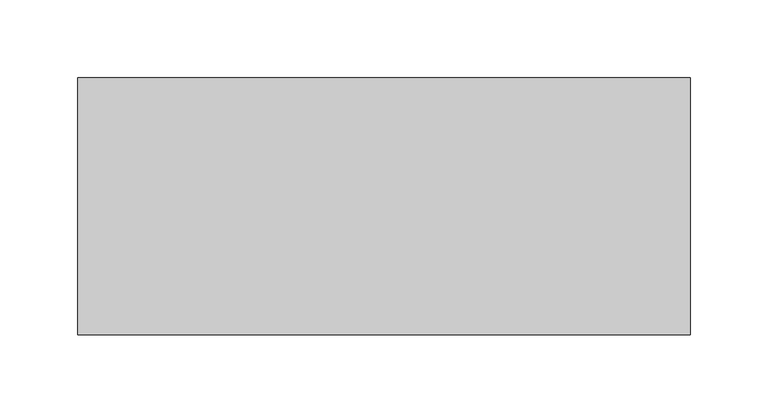
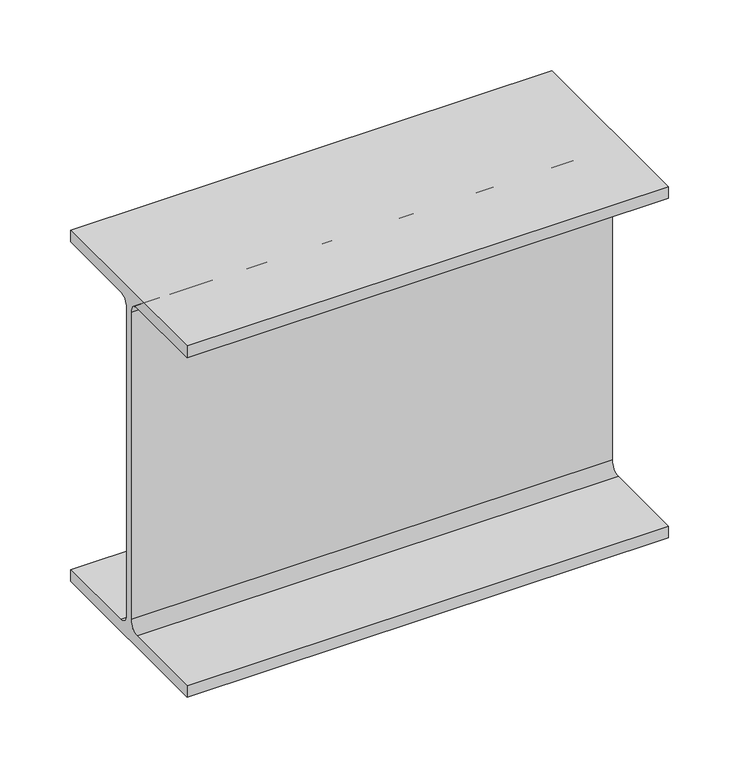
"""IFC4 building model written with IfcOpenShell, lengths in millimetres: beam geometry, Old_Steel Beam_H-KSD3502 : H_SB_ASB_H-300×150x6.5x9."""

from ifc_helpers import new_model, si_unit, point, frame, frame_2d, origin, place, context, project, spatial, polyline, circle_curve, trimmed, segment, composite_curve, outline, extrude, source, transform, mapped, element, save


def beam_0789f78f(model_context):
    return source(origin(), model_context, "Body", "SweptSolid", [
        extrude(outline(composite_curve([segment(polyline([(82.5, -141.5), (82.5, -151.7), (-82.5, -151.7), (-82.5, -141.5), (-11.9, -141.5)]), True, "CONTINUOUS"), segment(trimmed(circle_curve(frame_2d((-11.9, -132.6)), 8.9), [point((-11.9, -141.5))], [point((-3.0, -132.6))], True, "CARTESIAN"), True, "CONTINUOUS"), segment(polyline([(-3.0, -132.6), (-3.0, 132.6)]), True, "CONTINUOUS"), segment(trimmed(circle_curve(frame_2d((-11.9, 132.6)), 8.9), [point((-3.0, 132.6))], [point((-11.9, 141.5))], True, "CARTESIAN"), True, "CONTINUOUS"), segment(polyline([(-11.9, 141.5), (-82.5, 141.5), (-82.5, 151.7), (82.5, 151.7), (82.5, 141.5), (11.9, 141.5)]), True, "CONTINUOUS"), segment(trimmed(circle_curve(frame_2d((11.9, 132.6)), 8.9), [point((11.9, 141.5))], [point((3.0, 132.6))], True, "CARTESIAN"), True, "CONTINUOUS"), segment(polyline([(3.0, 132.6), (3.0, -132.6)]), True, "CONTINUOUS"), segment(trimmed(circle_curve(frame_2d((11.9, -132.6)), 8.9), [point((3.0, -132.6))], [point((11.9, -141.5))], True, "CARTESIAN"), True, "CONTINUOUS"), segment(polyline([(11.9, -141.5), (82.5, -141.5)]), True, "CONTINUOUS")], self_intersect=False)), frame((-190.2999994, 0.0, 0.0), z_axis=(1.0, 0.0, 0.0), x_axis=(0.0, 1.0, 0.0)), (0.0, 0.0, 1.0), 393.2999994),
    ])


if __name__ == "__main__":
    model = new_model("IFC4")
    model_context = context("Model", 3, world=origin())
    ifc_project = project(units=[si_unit("LENGTHUNIT", "METRE", prefix="MILLI")], contexts=[model_context])
    site = spatial("IfcSite", under=ifc_project)
    building = spatial("IfcBuilding", under=site)
    placement = place(None, origin())
    beam_shape = beam_0789f78f(model_context)
    element("IfcBeam", 1, ObjectType="Old_Steel Beam_H-KSD3502 : H_SB_ASB_H-300×150x6.5x9", at=placement, inside=building, context=model_context, shape_type="MappedRepresentation", body=[
        mapped(beam_shape, transform((0.0, 0.0, 0.0), x_axis=(1.0, 0.0, 0.0), y_axis=(0.0, 1.0, 0.0), z_axis=(0.0, 0.0, 1.0))),
    ])
    save(model, "model.ifc")

# Revit data of these elements
# Type "Old_Steel Beam_H-KSD3502 : H_SB_ASB_H-300×150x6.5x9"
#   Width = 15.0 cm
#   Web Thickness = 0.65 cm
#   Web Fillet = 1.3 cm
#   Warping Constant = 107174.0 cm⁶
#   Torsional Moment of Inertia = 9.9539 cm⁴
#   Torsional Modulus = 1.0 cm³
#   Section Area = 46.78 cm²
#   Plastic Modulus weak axis = 105.0 cm³
#   Plastic Modulus strong axis = 542.0 cm³
#   Perimeter = 1.17 m²/m
#   Nominal Weight = 36.70 kgf/m
#   Moment of Inertia weak axis = 508.00 cm⁴
#   Moment of Inertia strong axis = 7210.00 cm⁴
#   Height = 30.0 cm
#   Flange Thickness = 0.9 cm
#   Elastic Modulus weak axis = 67.7 cm³
#   Elastic Modulus strong axis = 481.0 cm³
#   Centroid Vertical = 15.0 cm
#   Centroid Horizontal = 7.5 cm
#   Length [instance default] = 1.5240 m
#   Structural Material [instance default] = Steel, 45-345
#   Assembly Code = ""
# Element 1 (IfcBeam, "Old_Steel Beam_H-KSD3502 : H_SB_ASB_H-300×150x6.5x9")
#   Structural Material = none
# Materials
#   "Steel, 45-345": class "Metal", colour RGB 189 187 185, transparency 0, Description = "Steel 345 MPa", Cost = 0
